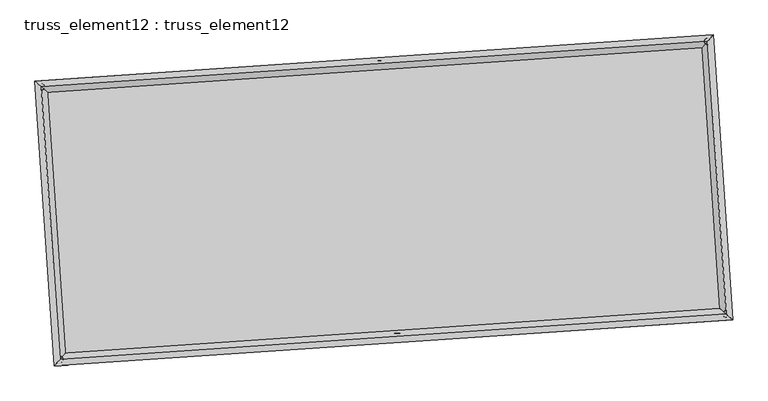
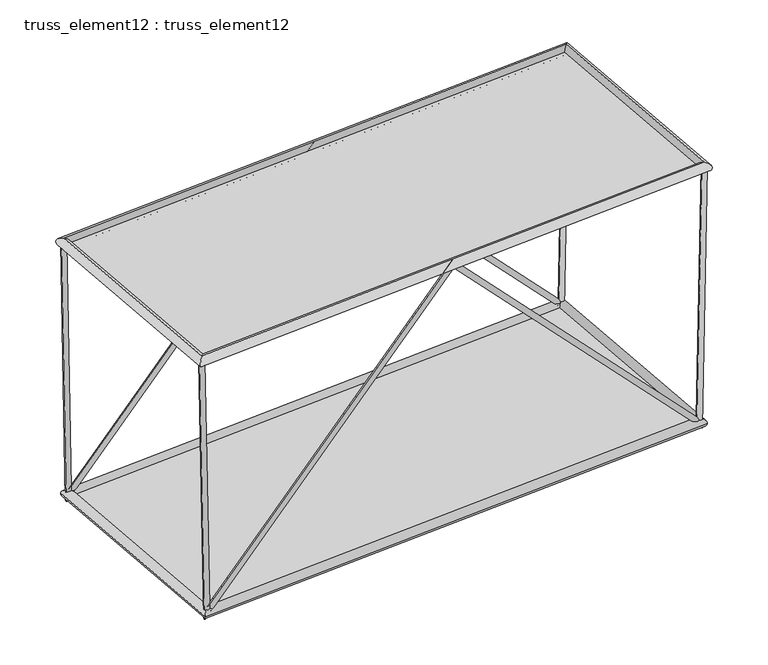
"""IFC4 building model written with IfcOpenShell, lengths in millimetres: plate geometry, truss_element12 : truss_element12."""

import ifcopenshell
import ifcopenshell.guid

model = None  # the IFC model being written
_history = None  # IfcOwnerHistory: only IFC2X3 demands one
_inside = {}  # id of a spatial element -> (the spatial element, [elements in it])
_under = {}  # id of a project, library or spatial element -> (it, [spatial elements below it])
_declared = {}  # id of a project -> (the project, [libraries it declares])
_typed = {}  # id of a type object -> (the type object, [elements of that type])
_made_of = {}  # id of a material, layer set ... -> (it, [elements and type objects made of it])


def new_model(schema):
    """Start an empty IFC model of exactly this schema.

    Asked for "IFC4X3", IfcOpenShell would pick the latest addendum, in which some entities
    have other attributes; the version numbers below select the first issue.
    IFC2X3 requires an IfcOwnerHistory on every rooted entity: one is made here for all.
    """
    global model, _history
    if schema == "IFC4X3":
        model = ifcopenshell.file(schema_version=(4, 3, 0, 0))
    else:
        model = ifcopenshell.file(schema=schema)
    _inside.clear()
    _under.clear()
    _declared.clear()
    _typed.clear()
    _made_of.clear()
    _history = None
    if model.schema == "IFC2X3":
        org = make("IfcOrganization", Name="unknown")
        user = make(
            "IfcPersonAndOrganization",
            ThePerson=make("IfcPerson", FamilyName="unknown"),
            TheOrganization=org,
        )
        app = make(
            "IfcApplication",
            ApplicationDeveloper=org,
            Version="unknown",
            ApplicationFullName="unknown",
            ApplicationIdentifier="unknown",
        )
        _history = make(
            "IfcOwnerHistory",
            OwningUser=user,
            OwningApplication=app,
            ChangeAction="ADDED",
            CreationDate=0,
        )
    return model


def make(cls, **values):
    """One entity of the class cls with the attributes given. An attribute that is None is left unset."""
    return model.create_entity(
        cls, **{name: value for name, value in values.items() if value is not None}
    )


def rooted(cls, **values):
    """An entity with a GlobalId (a new one), such as an element, a storey or a relation."""
    return make(cls, GlobalId=ifcopenshell.guid.new(), OwnerHistory=_history, **values)


def si_unit(unit_type, name, prefix=None):
    """IfcSIUnit, for example si_unit("LENGTHUNIT", "METRE", prefix="MILLI")."""
    return make("IfcSIUnit", UnitType=unit_type, Prefix=prefix, Name=name)


def assignment(units):
    """IfcUnitAssignment: the units of a project."""
    return None if units is None else make("IfcUnitAssignment", Units=units)


def point(xyz):
    """IfcCartesianPoint."""
    return None if xyz is None else make("IfcCartesianPoint", Coordinates=xyz)


def direction(xyz):
    """IfcDirection."""
    return None if xyz is None else make("IfcDirection", DirectionRatios=xyz)


def frame(location, z_axis=None, x_axis=None):
    """IfcAxis2Placement3D, a coordinate frame: its origin and axes. An axis left out is left unset."""
    return make(
        "IfcAxis2Placement3D",
        Location=point(location),
        Axis=direction(z_axis),
        RefDirection=direction(x_axis),
    )


def origin():
    """The frame at (0, 0, 0) with its axes left unset."""
    return frame((0.0, 0.0, 0.0))


def origin_with_axes():
    """The frame at (0, 0, 0) with the z axis (0, 0, 1) and the x axis (1, 0, 0) written out."""
    return frame((0.0, 0.0, 0.0), z_axis=(0.0, 0.0, 1.0), x_axis=(1.0, 0.0, 0.0))


def place(relative_to, where):
    """IfcLocalPlacement: puts the frame where relative to a parent placement (None: the world)."""
    return make(
        "IfcLocalPlacement", PlacementRelTo=relative_to, RelativePlacement=where
    )


def context(
    kind, dimensions, precision=None, world=None, true_north=None, identifier=None
):
    """IfcGeometricRepresentationContext, for example the 3D "Model" context."""
    return make(
        "IfcGeometricRepresentationContext",
        ContextIdentifier=identifier,
        ContextType=kind,
        CoordinateSpaceDimension=dimensions,
        Precision=precision,
        WorldCoordinateSystem=world,
        TrueNorth=true_north,
    )


def project(units=None, contexts=None):
    """IfcProject with its units and contexts."""
    return rooted(
        "IfcProject",
        Name="project",
        RepresentationContexts=contexts,
        UnitsInContext=assignment(units),
    )


def spatial(cls, under=None, at=None, **own):
    """A site, building, storey or space (cls), placed at a placement, below another one or the project."""
    s = rooted(cls, ObjectPlacement=at, **own)
    if under is not None:
        _under.setdefault(under.id(), (under, []))[1].append(s)
    return s


def polyline(points):
    """IfcPolyline through the points."""
    return make("IfcPolyline", Points=[point(p) for p in points])


def circle_curve(where, radius):
    """IfcCircle in the frame where."""
    return make("IfcCircle", Position=where, Radius=radius)


def ellipse_curve(where, semi_axis1, semi_axis2):
    """IfcEllipse in the frame where."""
    return make(
        "IfcEllipse", Position=where, SemiAxis1=semi_axis1, SemiAxis2=semi_axis2
    )


def outline(outer, holes=None, kind="AREA"):
    """IfcArbitraryClosedProfileDef: a profile drawn as a closed curve; with holes, ...WithVoids."""
    if holes is None:
        return make("IfcArbitraryClosedProfileDef", ProfileType=kind, OuterCurve=outer)
    return make(
        "IfcArbitraryProfileDefWithVoids",
        ProfileType=kind,
        OuterCurve=outer,
        InnerCurves=holes,
    )


def extrude(swept, where, along, depth):
    """IfcExtrudedAreaSolid: the profile swept, set in the frame where, extruded along a direction by depth."""
    return make(
        "IfcExtrudedAreaSolid",
        SweptArea=swept,
        Position=where,
        ExtrudedDirection=direction(along),
        Depth=depth,
    )


def shape(context_of_items, identifier, shape_type, items):
    """IfcShapeRepresentation: the items that make up one representation, for example the "Body"."""
    return make(
        "IfcShapeRepresentation",
        ContextOfItems=context_of_items,
        RepresentationIdentifier=identifier,
        RepresentationType=shape_type,
        Items=items,
    )


def source(mapping_origin, context_of_items, identifier, shape_type, items):
    """IfcRepresentationMap: a shape defined once, which mapped items show again and again."""
    return make(
        "IfcRepresentationMap",
        MappingOrigin=mapping_origin,
        MappedRepresentation=shape(context_of_items, identifier, shape_type, items),
    )


def transform(
    local_origin,
    x_axis=None,
    y_axis=None,
    z_axis=None,
    scale=None,
    scale2=None,
    scale3=None,
    uniform=True,
):
    """IfcCartesianTransformationOperator3D, or its non-uniform kind. x_axis, y_axis, z_axis: its Axis1, 2, 3."""
    if uniform:
        return make(
            "IfcCartesianTransformationOperator3D",
            Axis1=direction(x_axis),
            Axis2=direction(y_axis),
            LocalOrigin=point(local_origin),
            Scale=scale,
            Axis3=direction(z_axis),
        )
    return make(
        "IfcCartesianTransformationOperator3DnonUniform",
        Axis1=direction(x_axis),
        Axis2=direction(y_axis),
        LocalOrigin=point(local_origin),
        Scale=scale,
        Axis3=direction(z_axis),
        Scale2=scale2,
        Scale3=scale3,
    )


def mapped(mapping_source, mapping_target):
    """IfcMappedItem: shows the shape of a source again, moved by a transform."""
    return make(
        "IfcMappedItem", MappingSource=mapping_source, MappingTarget=mapping_target
    )


def made_of(thing, what):
    """Note that an element or type object is made of a material, layer set ...; save() writes the relation."""
    if what is not None:
        _made_of.setdefault(what.id(), (what, []))[1].append(thing)
    return thing


def element(
    cls,
    number,
    at=None,
    inside=None,
    cuts=None,
    type_object=None,
    material=None,
    context=None,
    identifier="Body",
    shape_type=None,
    held_by="IfcProductDefinitionShape",
    body=None,
    shapes=None,
    **own,
):
    """One element of the class cls, such as IfcWall. Its Tag is "e" and its number.

    at: its placement. inside: the storey or other place that contains it. cuts: it is an
    opening in that element (IfcRelVoidsElement). A single representation is given by context,
    identifier, shape_type and body (its items); several are given by shapes. held_by: the class
    of the entity that holds the representations. save() writes the other relations.
    """
    e = rooted(cls, Tag="e%d" % number, ObjectPlacement=at, **own)
    if body is not None:
        shapes = [shape(context, identifier, shape_type, body)]
    if shapes is not None:
        e.Representation = make(held_by, Representations=shapes)
    if inside is not None:
        _inside.setdefault(inside.id(), (inside, []))[1].append(e)
    if cuts is not None:
        rooted(
            "IfcRelVoidsElement", RelatingBuildingElement=cuts, RelatedOpeningElement=e
        )
    if type_object is not None:
        _typed.setdefault(type_object.id(), (type_object, []))[1].append(e)
    return made_of(e, material)


def aggregate(whole, parts):
    """IfcRelAggregates: a whole, such as a stair, and the parts it consists of."""
    return rooted("IfcRelAggregates", RelatingObject=whole, RelatedObjects=parts)


def save(model, path):
    """Write the relations noted so far, then the file.

    IfcRelAggregates (storeys below a building ...), IfcRelContainedInSpatialStructure (elements
    in a storey), IfcRelDefinesByType, IfcRelAssociatesMaterial and IfcRelDeclares: one each for
    every whole, place, type object, material and project.
    """
    for whole, parts in _under.values():
        aggregate(whole, parts)
    for where, things in _inside.values():
        rooted(
            "IfcRelContainedInSpatialStructure",
            RelatedElements=things,
            RelatingStructure=where,
        )
    for kind, things in _typed.values():
        rooted("IfcRelDefinesByType", RelatedObjects=things, RelatingType=kind)
    for what, things in _made_of.values():
        rooted("IfcRelAssociatesMaterial", RelatedObjects=things, RelatingMaterial=what)
    for by, libraries in _declared.values():
        rooted("IfcRelDeclares", RelatingContext=by, RelatedDefinitions=libraries)
    model.write(path)


def plane_surface(at):
    """IfcPlane: the flat surface through the origin of the frame at, square to its z axis."""
    return make("IfcPlane", Position=at)


def cylinder_surface(at, radius):
    """IfcCylindricalSurface: all points at the distance radius from the z axis of the frame at."""
    return make("IfcCylindricalSurface", Position=at, Radius=radius)


def advanced_brep(points, edges, surfaces, faces):
    """IfcAdvancedBrep: a solid bounded by faces that lie on surfaces and meet in shared edges.

    An edge is (start, end): straight between two places in points (the first is 0);
    or (start, end, curve); or (start, end, curve, False) where it runs against its curve.
    A face is (place in surfaces, loops), or (place, loops, False) where it looks against
    its surface's normal. A loop lists edges by number (the first is 1), with a minus sign
    where the edge is run from its end to its start. The first loop is the outer one.
    """
    corners = [point(p) for p in points]
    vertices = [make("IfcVertexPoint", VertexGeometry=c) for c in corners]
    made = []
    for start, end, *more in edges:
        made.append(
            make(
                "IfcEdgeCurve",
                EdgeStart=vertices[start],
                EdgeEnd=vertices[end],
                EdgeGeometry=more[0] if more else make("IfcPolyline", Points=[corners[start], corners[end]]),
                SameSense=more[1] if len(more) > 1 else True,
            )
        )
    hull = []
    for where, loops, *sense in faces:
        bounds = []
        for j, loop in enumerate(loops):
            ring = [make("IfcOrientedEdge", EdgeElement=made[abs(k) - 1], Orientation=k > 0) for k in loop]
            bounds.append(
                make(
                    "IfcFaceOuterBound" if j == 0 else "IfcFaceBound",
                    Bound=make("IfcEdgeLoop", EdgeList=ring),
                    Orientation=True,
                )
            )
        hull.append(make("IfcAdvancedFace", Bounds=bounds, FaceSurface=surfaces[where], SameSense=sense[0] if sense else True))
    return make("IfcAdvancedBrep", Outer=make("IfcClosedShell", CfsFaces=hull))


def truss_element12_truss_element12_8118c823(model_context):
    return source(origin(), model_context, "Body", "SolidModel", [
        advanced_brep(
        [(-3759.0101005, 2269.8097873, 5000.0518193), (-3858.0957712, 2256.449774, 4998.1703582), (-3667.2244266, 2276.0683035, 121.7906411), (-3761.7624562, 2263.0183766, -121.7906411), (1064.425668, 2598.7015368, 5071.2149108), (1064.8633229, 2592.1276407, 4926.9805686), (5794.6969904, 2921.2407568, 121.7809717), (5890.0639866, 2921.1397317, -121.7809717), (5887.8511571, 2927.5925853, 5000.0391427), (5987.8326962, 2927.8062083, 4998.1296386)],
        [
            (0, 1, circle_curve(frame((-3808.5529358, 2263.1297807, 4999.1110888), z_axis=(-0.018811898886610594, -0.001282711874355422, 0.9998222177519999), x_axis=(-0.13360051524293703, 0.9910344893322439, -0.0012422885334351164)), 50.0)),
            (1, 0, circle_curve(frame((-3808.5529358, 2263.1297807, 4999.1110888), z_axis=(-0.018811898886610594, -0.001282711874355422, 0.9998222177519999), x_axis=(-0.13360051524293703, 0.9910344893322439, -0.0012422885334351164)), 50.0)),
            (0, 2),
            (2, 3, ellipse_curve(frame((-3714.4934414, 2269.54334, 0.0), z_axis=(-0.9292247210951419, -0.06336030141761893, 0.3640424287221536), x_axis=(0.3631990866028644, 0.024765165066465387, 0.9313823651380112)), 131.0480431, 50.0)),
            (3, 1),
            (3, 2, ellipse_curve(frame((-3714.4934414, 2269.54334, 0.0), z_axis=(-0.9292247210951419, -0.06336030141761893, 0.3640424287221536), x_axis=(0.3631990866028644, 0.024765165066465387, 0.9313823651380112)), 131.0480431, 50.0)),
            (2, 4),
            (4, 5, ellipse_curve(frame((1064.6444954, 2595.4145888, 4999.0977397), z_axis=(-0.9976833933961031, -0.06802823804604483, 7.328019523198135e-05), x_axis=(-7.311043404423826e-05, -4.985122578868747e-06, -0.9999999973150066)), 72.2742041, 50.0)),
            (5, 3),
            (5, 4, ellipse_curve(frame((1064.6444954, 2595.4145888, 4999.0977397), z_axis=(-0.9976833933961031, -0.06802823804604483, 7.328019523198135e-05), x_axis=(-7.311043404423826e-05, -4.985122578868747e-06, -0.9999999973150066)), 72.2742041, 50.0)),
            (4, 6),
            (6, 7, ellipse_curve(frame((5842.3804885, 2921.1902443, 0.0), z_axis=(-0.9293023610631934, -0.06336559539190303, -0.3638432671398546), x_axis=(-0.3630003863990688, -0.024751616454898564, 0.9314601853847518)), 131.026691, 50.0)),
            (7, 5),
            (7, 6, ellipse_curve(frame((5842.3804885, 2921.1902443, 0.0), z_axis=(-0.9293023610631934, -0.06336559539190303, -0.3638432671398546), x_axis=(-0.3630003863990688, -0.024751616454898564, 0.9314601853847518)), 131.026691, 50.0)),
            (8, 9, circle_curve(frame((5937.8419267, 2927.6993968, 4999.0843906), z_axis=(0.019092287634230168, 0.001301830517198297, 0.9998168781282882), x_axis=(-0.002160697205567338, 0.9999968708746868, -0.0012608046719796988)), 50.0)),
            (9, 8, circle_curve(frame((5937.8419267, 2927.6993968, 4999.0843906), z_axis=(0.019092287634230168, 0.001301830517198297, 0.9998168781282882), x_axis=(-0.002160697205567338, 0.9999968708746868, -0.0012608046719796988)), 50.0)),
            (6, 8),
            (9, 7),
        ],
        [
            plane_surface(frame((-3808.5529358, 2313.1297395, 4999.1752357), z_axis=(-0.0188118988866116, -0.0012827118743585508, 0.9998222177519999), x_axis=(0.9998230405728206, -2.41345169111895e-05, 0.01881188340504991))),
            cylinder_surface(frame((-3808.5529358, 2263.1297807, 4999.1110888), z_axis=(-0.018811898886610594, -0.001282711874355422, 0.9998222177519999), x_axis=(-0.13360051524293703, 0.9910344893322439, -0.0012422885334351164)), 50.0),
            cylinder_surface(frame((-3714.4934414, 2269.54334, 0.0), z_axis=(-0.6902599032026427, -0.04706619887584547, -0.7220291122621425), x_axis=(-0.02042017886587182, 0.9987518262310586, -0.04558295619210198)), 50.0),
            cylinder_surface(frame((1064.6444954, 2595.4145888, 4999.0977397), z_axis=(-0.690154320065973, -0.04705899956311478, 0.7221305041710904), x_axis=(-0.11534734726939705, 0.9922791034695722, -0.04557598375828237)), 50.0),
            plane_surface(frame((5937.8419267, 2877.6994392, 4999.149494), z_axis=(0.019092287634229446, 0.0013018305172036945, 0.9998168781282883), x_axis=(0.9998177256644792, -2.485945392649572e-05, -0.01909227144987471))),
            cylinder_surface(frame((5842.3804885, 2921.1902443, 0.0), z_axis=(-0.019092287634230168, -0.001301830517198297, -0.9998168781282882), x_axis=(-0.002160697205567338, 0.9999968708746868, -0.0012608046719796988)), 50.0),
        ],
        [
            (0, [[1, 2]]),
            (1, [[-1, 3, 4, 5]]),
            (1, [[-2, -5, 6, -3]]),
            (2, [[-4, 7, 8, 9]]),
            (2, [[-6, -9, 10, -7]]),
            (3, [[-8, 11, 12, 13]]),
            (3, [[-10, -13, 14, -11]]),
            (4, [[15, 16]]),
            (5, [[-12, 17, -16, 18]]),
            (5, [[-14, -18, -15, -17]]),
        ],
    ),
        advanced_brep(
        [(-3486.8971476, -1720.923797, 5000.0518193), (-3585.9828183, -1734.2838103, 4998.1703582), (-3395.1114737, -1714.6652808, 121.7906411), (-3489.6495033, -1727.7152077, -121.7906411), (1336.5386209, -1392.0320475, 5071.2149108), (1336.9762758, -1398.6059436, 4926.9805686), (6066.8099433, -1069.4928275, 121.7809717), (6162.1769395, -1069.5938526, -121.7809717), (6159.96411, -1063.140999, 5000.0391427), (6259.9456491, -1062.927376, 4998.1296386)],
        [
            (0, 1, circle_curve(frame((-3536.4399829, -1727.6038036, 4999.1110888), z_axis=(-0.018811898886610712, -0.0012827118743554558, 0.999822217752), x_axis=(-0.13360051524293726, 0.9910344893322439, -0.0012422885334351028)), 50.0)),
            (1, 0, circle_curve(frame((-3536.4399829, -1727.6038036, 4999.1110888), z_axis=(-0.018811898886610712, -0.0012827118743554558, 0.999822217752), x_axis=(-0.13360051524293726, 0.9910344893322439, -0.0012422885334351028)), 50.0)),
            (0, 2),
            (2, 3, ellipse_curve(frame((-3442.3804885, -1721.1902443, 0.0), z_axis=(-0.9292247210951418, -0.0633603014176191, 0.3640424287221536), x_axis=(0.3631990866028643, 0.02476516506646543, 0.9313823651380113)), 131.0480431, 50.0)),
            (3, 1),
            (3, 2, ellipse_curve(frame((-3442.3804885, -1721.1902443, 0.0), z_axis=(-0.9292247210951418, -0.0633603014176191, 0.3640424287221536), x_axis=(0.3631990866028643, 0.02476516506646543, 0.9313823651380113)), 131.0480431, 50.0)),
            (2, 4),
            (4, 5, ellipse_curve(frame((1336.7574483, -1395.3189955, 4999.0977397), z_axis=(-0.9976833933961031, -0.06802823804604513, 7.328019523166036e-05), x_axis=(-7.311043404393078e-05, -4.985122578705386e-06, -0.9999999973150066)), 72.2742041, 50.0)),
            (5, 3),
            (5, 4, ellipse_curve(frame((1336.7574483, -1395.3189955, 4999.0977397), z_axis=(-0.9976833933961031, -0.06802823804604513, 7.328019523166036e-05), x_axis=(-7.311043404393078e-05, -4.985122578705386e-06, -0.9999999973150066)), 72.2742041, 50.0)),
            (4, 6),
            (6, 7, ellipse_curve(frame((6114.4934414, -1069.54334, 0.0), z_axis=(-0.9293023610631932, -0.06336559539190349, -0.36384326713985504), x_axis=(-0.36300038639906934, -0.024751616454898748, 0.9314601853847516)), 131.026691, 50.0)),
            (7, 5),
            (7, 6, ellipse_curve(frame((6114.4934414, -1069.54334, 0.0), z_axis=(-0.9293023610631932, -0.06336559539190349, -0.36384326713985504), x_axis=(-0.36300038639906934, -0.024751616454898748, 0.9314601853847516)), 131.026691, 50.0)),
            (8, 9, circle_curve(frame((6209.9548796, -1063.0341875, 4999.0843906), z_axis=(0.019092287634229887, 0.0013018305171983192, 0.9998168781282882), x_axis=(-0.002160697205567476, 0.9999968708746868, -0.0012608046719797192)), 50.0)),
            (9, 8, circle_curve(frame((6209.9548796, -1063.0341875, 4999.0843906), z_axis=(0.019092287634229887, 0.0013018305171983192, 0.9998168781282882), x_axis=(-0.002160697205567476, 0.9999968708746868, -0.0012608046719797192)), 50.0)),
            (6, 8),
            (9, 7),
        ],
        [
            plane_surface(frame((-3536.4399829, -1677.6038448, 4999.1752357), z_axis=(-0.0188118988866116, -0.0012827118743585543, 0.9998222177519999), x_axis=(0.9998230405728206, -2.41345169111895e-05, 0.01881188340504991))),
            cylinder_surface(frame((-3536.4399829, -1727.6038036, 4999.1110888), z_axis=(-0.01881189888661071, -0.0012827118743554556, 0.9998222177519998), x_axis=(-0.13360051524293726, 0.9910344893322439, -0.0012422885334351028)), 50.0),
            cylinder_surface(frame((-3442.3804885, -1721.1902443, 0.0), z_axis=(-0.6902599032026429, -0.04706619887584558, -0.7220291122621424), x_axis=(-0.020420178865871896, 0.9987518262310586, -0.045582956192102064)), 50.0),
            cylinder_surface(frame((1336.7574483, -1395.3189955, 4999.0977397), z_axis=(-0.6901543200659735, -0.04705899956311514, 0.72213050417109), x_axis=(-0.11534734726939751, 0.9922791034695722, -0.04557598375828241)), 50.0),
            plane_surface(frame((6209.9548796, -1113.0341451, 4999.149494), z_axis=(0.019092287634229446, 0.001301830517192873, 0.9998168781282883), x_axis=(0.9998177256644792, -2.485945392560754e-05, -0.01909227144987471))),
            cylinder_surface(frame((6114.4934414, -1069.54334, 0.0), z_axis=(-0.019092287634229887, -0.0013018305171983192, -0.9998168781282882), x_axis=(-0.002160697205567476, 0.9999968708746868, -0.0012608046719797192)), 50.0),
        ],
        [
            (0, [[1, 2]]),
            (1, [[-1, 3, 4, 5]]),
            (1, [[-2, -5, 6, -3]]),
            (2, [[-4, 7, 8, 9]]),
            (2, [[-6, -9, 10, -7]]),
            (3, [[-8, 11, 12, 13]]),
            (3, [[-10, -13, 14, -11]]),
            (4, [[15, 16]]),
            (5, [[-12, 17, -16, 18]]),
            (5, [[-14, -18, -15, -17]]),
        ],
    ),
        advanced_brep(
        [(-3536.4469431, -1727.6115178, 4909.1110891), (-3536.4330228, -1727.5960894, 5089.1110885), (-3808.544993, 2263.1230826, 5089.1110885), (-3808.5608787, 2263.1364787, 4909.1110891), (5937.8354573, 2927.6917161, 5089.0843904), (5937.848396, 2927.7070776, 4909.0843909), (6209.9474275, -1063.027456, 5089.0843904), (6209.9623317, -1063.040919, 4909.0843909)],
        [
            (0, 1, ellipse_curve(frame((-3536.4399829, -1727.6038036, 4999.1110888), z_axis=(-0.7535719234028208, 0.6573654662782634, 1.932477302402373e-06), x_axis=(-0.6573654662754491, -0.7535719234052757, 1.932477302785358e-06)), 127.2792206, 90.0)),
            (1, 2),
            (2, 3, ellipse_curve(frame((-3808.5529358, 2263.1297807, 4999.1110888), z_axis=(-0.6573654662754492, -0.7535719234052756, 1.93247730270711e-06), x_axis=(0.7535719234028205, -0.6573654662782638, -1.9324773023241237e-06)), 127.2792206, 90.0)),
            (3, 0),
            (1, 0, ellipse_curve(frame((-3536.4399829, -1727.6038036, 4999.1110888), z_axis=(-0.7535719234028208, 0.6573654662782634, 1.932477302402373e-06), x_axis=(-0.6573654662754491, -0.7535719234052757, 1.932477302785358e-06)), 127.2792206, 90.0)),
            (3, 2, ellipse_curve(frame((-3808.5529358, 2263.1297807, 4999.1110888), z_axis=(-0.6573654662754492, -0.7535719234052756, 1.93247730270711e-06), x_axis=(0.7535719234028205, -0.6573654662782638, -1.9324773023241237e-06)), 127.2792206, 90.0)),
            (2, 4),
            (4, 5, ellipse_curve(frame((5937.8419267, 2927.6993968, 4999.0843906), z_axis=(-0.7535719234028213, 0.6573654662782629, 1.932477302515678e-06), x_axis=(-0.6573654662754486, -0.7535719234052763, 1.932477302515556e-06)), 127.2792206, 90.0)),
            (5, 3),
            (5, 4, ellipse_curve(frame((5937.8419267, 2927.6993968, 4999.0843906), z_axis=(-0.7535719234028213, 0.6573654662782629, 1.932477302515678e-06), x_axis=(-0.6573654662754486, -0.7535719234052763, 1.932477302515556e-06)), 127.2792206, 90.0)),
            (4, 6),
            (6, 7, ellipse_curve(frame((6209.9548796, -1063.0341875, 4999.0843906), z_axis=(0.6573654662754486, 0.7535719234052763, -1.932477302593805e-06), x_axis=(-0.7535719234028213, 0.6573654662782628, 1.932477302593927e-06)), 127.2792206, 90.0)),
            (7, 5),
            (7, 6, ellipse_curve(frame((6209.9548796, -1063.0341875, 4999.0843906), z_axis=(0.6573654662754486, 0.7535719234052763, -1.932477302593805e-06), x_axis=(-0.7535719234028213, 0.6573654662782628, 1.932477302593927e-06)), 127.2792206, 90.0)),
            (6, 1),
            (0, 7),
        ],
        [
            cylinder_surface(frame((-3536.4399829, -1727.6038036, 4999.1110888), z_axis=(0.06802823822869636, -0.997683396074877, 0.0), x_axis=(-0.997683392639436, -0.0680282379944467, 8.298696282030801e-05)), 90.0),
            cylinder_surface(frame((-3808.5529358, 2263.1297807, 4999.1110888), z_axis=(-0.997683396071151, -0.06802823822844395, 2.7329356101957602e-06), x_axis=(-0.06802823779080196, 0.9976833928769032, 8.025402721864263e-05)), 90.0),
            cylinder_surface(frame((5937.8419267, 2927.6993968, 4999.0843906), z_axis=(-0.06802823822869826, 0.997683396074877, 0.0), x_axis=(0.9976833930770779, 0.06802823802428974, 7.752109161724803e-05)), 90.0),
            cylinder_surface(frame((6209.9548796, -1063.0341875, 4999.0843906), z_axis=(0.997683396071151, 0.06802823822844414, -2.7329356103064204e-06), x_axis=(0.06802823822844414, -0.9976833928470621, 8.025402721875352e-05)), 90.0),
        ],
        [
            (0, [[1, 2, 3, 4]]),
            (0, [[5, -4, 6, -2]]),
            (1, [[-3, 7, 8, 9]]),
            (1, [[-6, -9, 10, -7]]),
            (2, [[-8, 11, 12, 13]]),
            (2, [[-10, -13, 14, -11]]),
            (3, [[-12, 15, -1, 16]]),
            (3, [[-14, -16, -5, -15]]),
        ],
    ),
        advanced_brep(
        [(-3358.7115243, -1625.2761972, 0.0), (-3526.0494527, -1817.1042913, 0.0), (-3810.4074885, 2353.2123043, 0.0), (-3618.5793943, 2185.8743758, 0.0), (5926.0494527, 3017.1042913, 0.0), (5758.7115243, 2825.2761972, 0.0), (6210.4074885, -1153.2123043, 0.0), (6018.5793943, -985.8743758, 0.0)],
        [
            (0, 1, ellipse_curve(frame((-3442.3804885, -1721.1902443, 0.0), z_axis=(-0.7535719234054569, 0.6573654662780819, 0.0), x_axis=(-0.6573654662780818, -0.7535719234054571, 0.0)), 127.2792206, 90.0)),
            (1, 2),
            (2, 3, ellipse_curve(frame((-3714.4934414, 2269.54334, 0.0), z_axis=(-0.6573654662780819, -0.753571923405457, 0.0), x_axis=(0.7535719234054569, -0.6573654662780819, 0.0)), 127.2792206, 90.0)),
            (3, 0),
            (1, 0, ellipse_curve(frame((-3442.3804885, -1721.1902443, 0.0), z_axis=(-0.7535719234054569, 0.6573654662780819, 0.0), x_axis=(-0.6573654662780818, -0.7535719234054571, 0.0)), 127.2792206, 90.0)),
            (3, 2, ellipse_curve(frame((-3714.4934414, 2269.54334, 0.0), z_axis=(-0.6573654662780819, -0.753571923405457, 0.0), x_axis=(0.7535719234054569, -0.6573654662780819, 0.0)), 127.2792206, 90.0)),
            (2, 4),
            (4, 5, ellipse_curve(frame((5842.3804885, 2921.1902443, 0.0), z_axis=(-0.7535719234054578, 0.657365466278081, 0.0), x_axis=(-0.657365466278081, -0.7535719234054576, 0.0)), 127.2792206, 90.0)),
            (5, 3),
            (5, 4, ellipse_curve(frame((5842.3804885, 2921.1902443, 0.0), z_axis=(-0.7535719234054578, 0.657365466278081, 0.0), x_axis=(-0.657365466278081, -0.7535719234054576, 0.0)), 127.2792206, 90.0)),
            (4, 6),
            (6, 7, ellipse_curve(frame((6114.4934414, -1069.54334, 0.0), z_axis=(0.6573654662780811, 0.7535719234054576, 0.0), x_axis=(-0.7535719234054576, 0.6573654662780812, 0.0)), 127.2792206, 90.0)),
            (7, 5),
            (7, 6, ellipse_curve(frame((6114.4934414, -1069.54334, 0.0), z_axis=(0.6573654662780811, 0.7535719234054576, 0.0), x_axis=(-0.7535719234054576, 0.6573654662780812, 0.0)), 127.2792206, 90.0)),
            (6, 1),
            (0, 7),
        ],
        [
            cylinder_surface(frame((-3442.3804885, -1721.1902443, 0.0), z_axis=(0.06802823822869888, -0.9976833960748768, 0.0), x_axis=(-0.9976833960748768, -0.06802823822869888, 0.0)), 90.0),
            cylinder_surface(frame((-3714.4934414, 2269.54334, 0.0), z_axis=(-0.9976833960748767, -0.06802823822870076, 0.0), x_axis=(-0.06802823822870076, 0.9976833960748767, 0.0)), 90.0),
            cylinder_surface(frame((5842.3804885, 2921.1902443, 0.0), z_axis=(-0.06802823822870105, 0.9976833960748767, 0.0), x_axis=(0.9976833960748767, 0.06802823822870105, 0.0)), 90.0),
            cylinder_surface(frame((6114.4934414, -1069.54334, 0.0), z_axis=(0.9976833960748767, 0.06802823822870052, 0.0), x_axis=(0.06802823822870052, -0.9976833960748767, 0.0)), 90.0),
        ],
        [
            (0, [[1, 2, 3, 4]]),
            (0, [[5, -4, 6, -2]]),
            (1, [[-3, 7, 8, 9]]),
            (1, [[-6, -9, 10, -7]]),
            (2, [[-8, 11, 12, 13]]),
            (2, [[-10, -13, 14, -11]]),
            (3, [[-12, 15, -1, 16]]),
            (3, [[-14, -16, -5, -15]]),
        ],
    ),
        extrude(outline(polyline([(-3442.3804885, -1721.1902443), (-3714.4934414, 2269.54334), (5842.3804885, 2921.1902443), (6114.4934414, -1069.54334), (-3442.3804885, -1721.1902443)])), origin_with_axes(), (0.0, 0.0, 1.0), 20.0),
        extrude(outline(polyline([(-2000.0, 4884.5129131), (2000.0, 4884.512913), (2000.0, -4884.5129131), (-2000.0, -4884.512913), (-2000.0, 4884.5129131)])), frame((1200.7009719, 600.0477966, 4999.0977397), z_axis=(2.726604480815564e-06, 1.8591679502417433e-07, 0.9999999999962655), x_axis=(-0.06802823822869859, 0.9976833960748768, 0.0)), (0.0, 0.0, 1.0), 20.0),
    ])


if __name__ == "__main__":
    model = new_model("IFC4")
    model_context = context("Model", 3, world=origin())
    ifc_project = project(units=[si_unit("LENGTHUNIT", "METRE", prefix="MILLI")], contexts=[model_context])
    site = spatial("IfcSite", under=ifc_project)
    building = spatial("IfcBuilding", under=site)
    placement = place(None, origin())
    truss_element12_truss_element12_shape = truss_element12_truss_element12_8118c823(model_context)
    element("IfcPlate", 1, ObjectType="truss_element12 : truss_element12", at=placement, inside=building, context=model_context, shape_type="MappedRepresentation", body=[
        mapped(truss_element12_truss_element12_shape, transform((0.0, 0.0, 0.0), x_axis=(1.0, 0.0, 0.0), y_axis=(0.0, 1.0, 0.0), z_axis=(0.0, 0.0, 1.0))),
    ])
    save(model, "model.ifc")

# Revit data of these elements
# Type "truss_element12 : truss_element12"
#   steellbar1 = 90 mm
#   steelbar2 = 50 mm
#   offset1 = 5000 mm
#   M = Default Roof
# Element 1 (IfcPlate, "truss_element12 : truss_element12")
#   Materials on its faces: "Default Roof"
# Materials
#   "Default Roof": class "Miscellaneous", colour RGB 0 127 0, transparency 0, Comments = "Rendering appearance not upgraded Rendering appearance not upgraded ", Cost = 0
